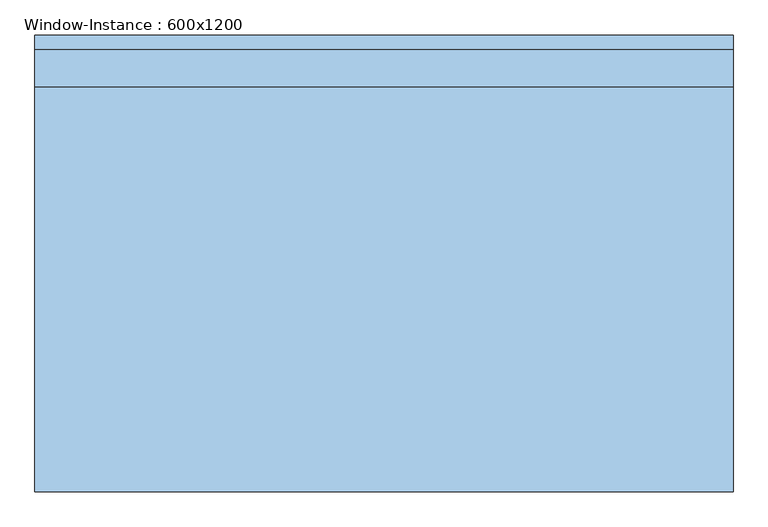
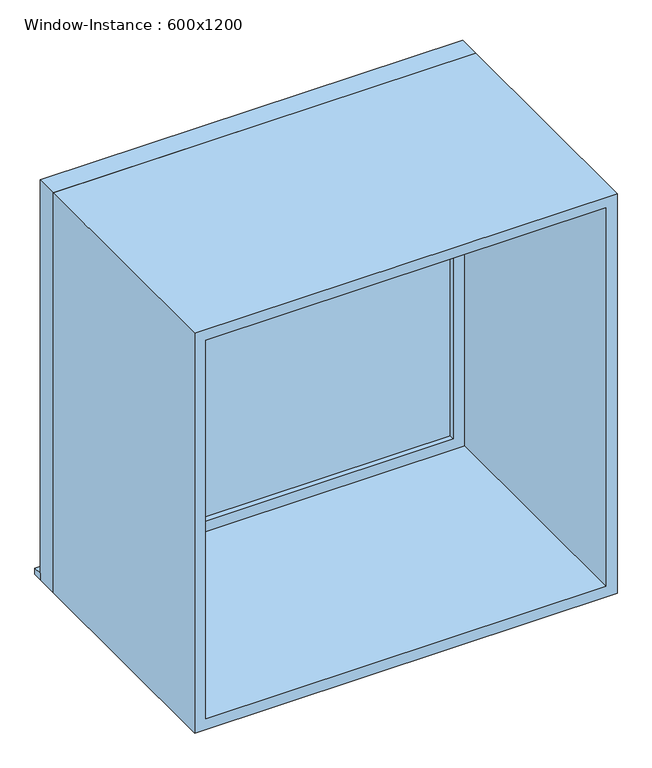
"""IFC4 building model written with IfcOpenShell, lengths in millimetres: window geometry, Window-Instance : 600x1200."""

from ifc_helpers import new_model, si_unit, frame, origin, place, context, project, spatial, polyline, outline, extrude, source, transform, mapped, element, save


def window_instance_600x1200_de133162(model_context):
    return source(origin(), model_context, "Body", "SweptSolid", [
        extrude(outline(polyline([(-638.1, 405.4), (561.9, 405.4), (561.9, 380.0), (-638.1, 380.0), (-638.1, 405.4)])), frame((0.0, 0.0, 900.0), z_axis=(0.0, 0.0, 1.0), x_axis=(1.0, 0.0, 0.0)), (0.0, 0.0, 1.0), 19.05),
        extrude(outline(polyline([(498.4, 331.425), (-574.6, 331.425), (-574.6, 344.125), (498.4, 344.125), (498.4, 331.425)])), frame((0.0, 0.0, 963.5), z_axis=(0.0, 0.0, 1.0), x_axis=(1.0, 0.0, 0.0)), (0.0, 0.0, 1.0), 1073.0),
        extrude(outline(polyline([(2080.95, -619.05), (919.05, -619.05), (919.05, 542.85), (2080.95, 542.85), (2080.95, -619.05)]), holes=[polyline([(2036.5, -574.6), (2036.5, 498.4), (963.5, 498.4), (963.5, -574.6), (2036.5, -574.6)])]), frame((0.0, 315.55, 0.0), z_axis=(0.0, 1.0, 0.0), x_axis=(0.0, 0.0, 1.0)), (0.0, 0.0, 1.0), 44.45),
        extrude(outline(polyline([(2100.0, -638.1), (900.0, -638.1), (900.0, 561.9), (2100.0, 561.9), (2100.0, -638.1)]), holes=[polyline([(2068.25, -606.35), (2068.25, 530.15), (931.75, 530.15), (931.75, -606.35), (2068.25, -606.35)])]), frame((0.0, -380.0, 0.0), z_axis=(0.0, 1.0, 0.0), x_axis=(0.0, 0.0, 1.0)), (0.0, 0.0, 1.0), 695.55),
        extrude(outline(polyline([(2100.0, 561.9), (2100.0, -638.1), (900.0, -638.1), (900.0, 561.9), (2100.0, 561.9)]), holes=[polyline([(2080.95, 542.85), (919.05, 542.85), (919.05, -619.05), (2080.95, -619.05), (2080.95, 542.85)])]), frame((0.0, 315.55, 0.0), z_axis=(0.0, 1.0, 0.0), x_axis=(0.0, 0.0, 1.0)), (0.0, 0.0, 1.0), 64.45),
    ])


if __name__ == "__main__":
    model = new_model("IFC4")
    model_context = context("Model", 3, world=origin())
    ifc_project = project(units=[si_unit("LENGTHUNIT", "METRE", prefix="MILLI")], contexts=[model_context])
    site = spatial("IfcSite", under=ifc_project)
    building = spatial("IfcBuilding", under=site)
    placement = place(None, origin())
    window_instance_600x1200_shape = window_instance_600x1200_de133162(model_context)
    element("IfcWindow", 1, ObjectType="Window-Instance : 600x1200", at=placement, inside=building, context=model_context, shape_type="MappedRepresentation", body=[
        mapped(window_instance_600x1200_shape, transform((0.0, 0.0, 0.0), x_axis=(1.0, 0.0, 0.0), y_axis=(0.0, 1.0, 0.0), z_axis=(0.0, 0.0, 1.0))),
    ])
    save(model, "model.ifc")

# Revit data of these elements
# Type "Window-Instance : 600x1200"
#   Type Mark = "7"
#   Construction Type Id = "GSP4R"
#   Assembly Code = "B2020100"
#   Analytic Construction = "1/8 in Pilkington single glazing"
#   Visual Light Transmittance = 0.9
#   Thermal Resistance (R) = 0.149095 (m²·K)/W
#   Solar Heat Gain Coefficient = 0.86
#   Heat Transfer Coefficient (U) = 6.70716 W/(m²·K)
#   Height [instance default] = 1200 mm
#   Default Sill Height = 900 mm
#   Width [instance default] = 600 mm
#   Window Inset = 20 mm
#   Glass Pane Material = WW-EC-GL-Storefront
#   Sash Material = WW-EC-RGB-White
#   Wall Closure = (empty or 0)
# Element 1 (IfcWindow, "Window-Instance : 600x1200")
#   Width = 1200 mm
#   Materials on its faces: "WW-EC-RGB-White", "WW-EC-GL-Storefront"
# Materials
#   "WW-EC-GL-Storefront": class "Glass", colour RGB 236 240 239, transparency 0.85, Description = "Storefront Glass", Cost = 0
#   "WW-EC-RGB-White": class "Generic", colour RGB 255 255 255, transparency 0, Comments = "If region requests off-white, swith asset color to RGB 231-228-220", Description = "Generic Color", Cost = 0
